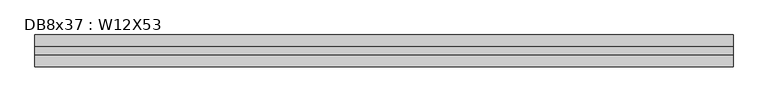
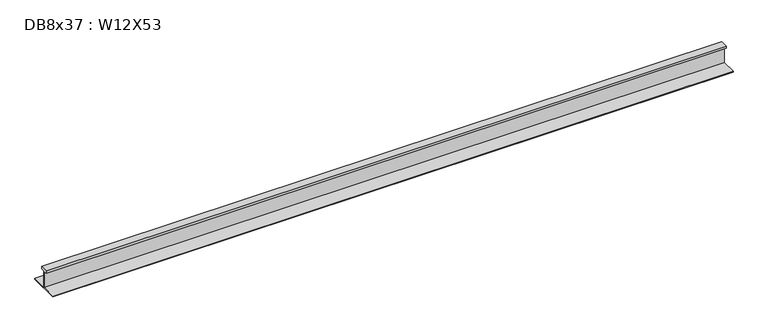
"""IFC4 building model written with IfcOpenShell, lengths in millimetres: beam geometry, DB8x37 : W12X53."""

from ifc_helpers import new_model, si_unit, frame, origin, place, context, project, spatial, polyline, outline, extrude, source, transform, mapped, element, save


def db8x37_w12x53_d28cac48(model_context):
    return source(origin(), model_context, "Body", "SweptSolid", [
        extrude(outline(polyline([(38.1, 145.415), (38.1, 120.015), (2.921, 120.015), (2.921, -48.4505), (152.4, -48.4505), (152.4, -58.1025), (-152.4, -58.1025), (-152.4, -48.4505), (-2.921, -48.4505), (-2.921, 120.015), (-38.1, 120.015), (-38.1, 145.415), (38.1, 145.415)])), frame((-3338.83, 0.0, 0.0), z_axis=(1.0, 0.0, 0.0), x_axis=(0.0, 1.0, 0.0)), (0.0, 0.0, 1.0), 6701.5687679),
    ])


if __name__ == "__main__":
    model = new_model("IFC4")
    model_context = context("Model", 3, world=origin())
    ifc_project = project(units=[si_unit("LENGTHUNIT", "METRE", prefix="MILLI")], contexts=[model_context])
    site = spatial("IfcSite", under=ifc_project)
    building = spatial("IfcBuilding", under=site)
    placement = place(None, origin())
    db8x37_w12x53_shape = db8x37_w12x53_d28cac48(model_context)
    element("IfcBeam", 1, ObjectType="DB8x37 : W12X53", at=placement, inside=building, context=model_context, shape_type="MappedRepresentation", body=[
        mapped(db8x37_w12x53_shape, transform((0.0, 0.0, 0.0), x_axis=(1.0, 0.0, 0.0), y_axis=(0.0, 1.0, 0.0), z_axis=(0.0, 0.0, 1.0))),
    ])
    save(model, "model.ifc")

# Revit data of these elements
# Type "DB8x37 : W12X53"
#   Assembly Code = "B10"
#   W = 53
#   Length [instance default] = 5' - 0"
#   bf = 0' - 10"
#   d = 1' - 0.1"
#   k = 0' - 1 3/8"
#   k2 = 0' - 0.8"
#   tf = 0' - 0.575"
#   tw = 0' - 0.345"
#   A = 0.108333 SF
#   Structural Material [instance default] = Steel ASTM A992
# Element 1 (IfcBeam, "DB8x37 : W12X53")
#   Materials on its faces: "Steel ASTM A992"
# Materials
#   "Steel ASTM A992": class "Metal", colour RGB 199 199 199, transparency 0, Description = "Structural steel 50ksi", Cost = 0
